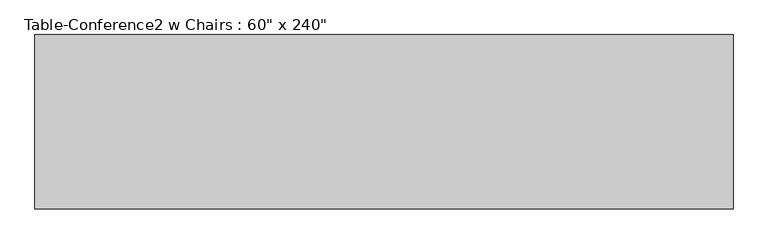
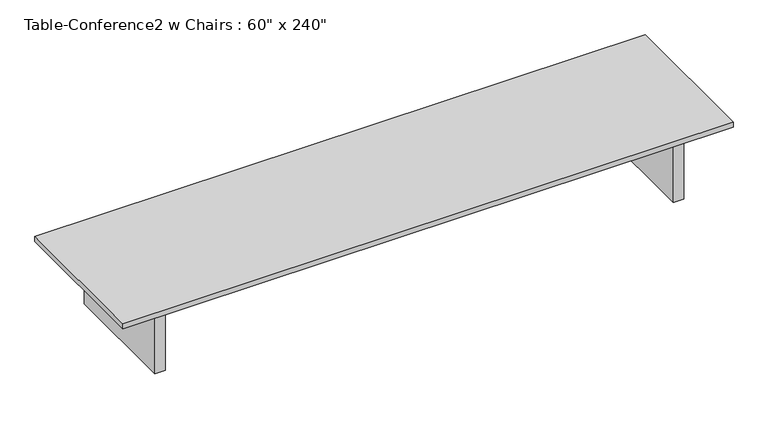
"""IFC4 building model written with IfcOpenShell, lengths in millimetres: furniture geometry."""

from ifc_helpers import new_model, si_unit, frame, origin, origin_with_axes, place, context, project, spatial, polyline, outline, extrude, source, transform, mapped, element, save


def furniture_b1813a45(model_context):
    return source(origin(), model_context, "Body", "SweptSolid", [
        extrude(outline(polyline([(2540.0, 609.6), (2540.0, 571.5), (-2540.0, 571.5), (-2540.0, 609.6), (2540.0, 609.6)])), frame((0.0, 0.0, 609.6), z_axis=(0.0, 0.0, 1.0), x_axis=(1.0, 0.0, 0.0)), (0.0, 0.0, 1.0), 101.6),
        extrude(outline(polyline([(2540.0, -609.6), (-2540.0, -609.6), (-2540.0, -571.5), (2540.0, -571.5), (2540.0, -609.6)])), frame((0.0, 0.0, 609.6), z_axis=(0.0, 0.0, 1.0), x_axis=(1.0, 0.0, 0.0)), (0.0, 0.0, 1.0), 101.6),
        extrude(outline(polyline([(-2540.0, -609.6), (-2641.6, -609.6), (-2641.6, 609.6), (-2540.0, 609.6), (-2540.0, -609.6)])), origin_with_axes(), (0.0, 0.0, 1.0), 711.2),
        extrude(outline(polyline([(2641.6, -609.6), (2540.0, -609.6), (2540.0, 609.6), (2641.6, 609.6), (2641.6, -609.6)])), origin_with_axes(), (0.0, 0.0, 1.0), 711.2),
        extrude(outline(polyline([(3048.0, -762.0), (-3048.0, -762.0), (-3048.0, 762.0), (3048.0, 762.0), (3048.0, -762.0)])), frame((0.0, 0.0, 711.2), z_axis=(0.0, 0.0, 1.0), x_axis=(1.0, 0.0, 0.0)), (0.0, 0.0, 1.0), 50.8),
    ])


if __name__ == "__main__":
    model = new_model("IFC4")
    model_context = context("Model", 3, world=origin())
    ifc_project = project(units=[si_unit("LENGTHUNIT", "METRE", prefix="MILLI")], contexts=[model_context])
    site = spatial("IfcSite", under=ifc_project)
    building = spatial("IfcBuilding", under=site)
    placement = place(None, origin())
    furniture_shape = furniture_b1813a45(model_context)
    element("IfcFurniture", 1, ObjectType="Table-Conference2 w Chairs : 60\" x 240\"", at=placement, inside=building, context=model_context, shape_type="MappedRepresentation", body=[
        mapped(furniture_shape, transform((0.0, 0.0, 0.0), x_axis=(1.0, 0.0, 0.0), y_axis=(0.0, 1.0, 0.0), z_axis=(0.0, 0.0, 1.0))),
    ])
    save(model, "model.ifc")

# Revit data of these elements
# Type "Table-Conference2 w Chairs : 60\" x 240\""
#   Type IfcGUID = "2u0XNFrAPALBFZCv81fqiU"
#   Assembly Code = "E2020200"
#   Description = "Seating 20-22"
#   Height = 0.762 m
#   Length = 6.096 m
#   Width = 1.524 m
#   Number Of Chairs One Side = 9
#   Number Of Chairs = 20
#   Material = Wood - Cherry
#   Default Elevation = 0
# Element 1 (IfcFurniture, "Table-Conference2 w Chairs : 60\" x 240\"")
#   Materials on its faces: "Wood - Cherry"
# Materials
#   "Wood - Cherry": class "Wood", colour RGB 226 177 128, transparency 0
